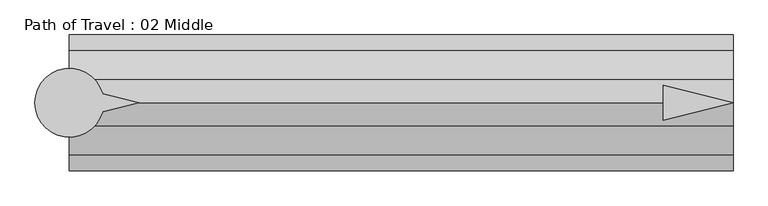
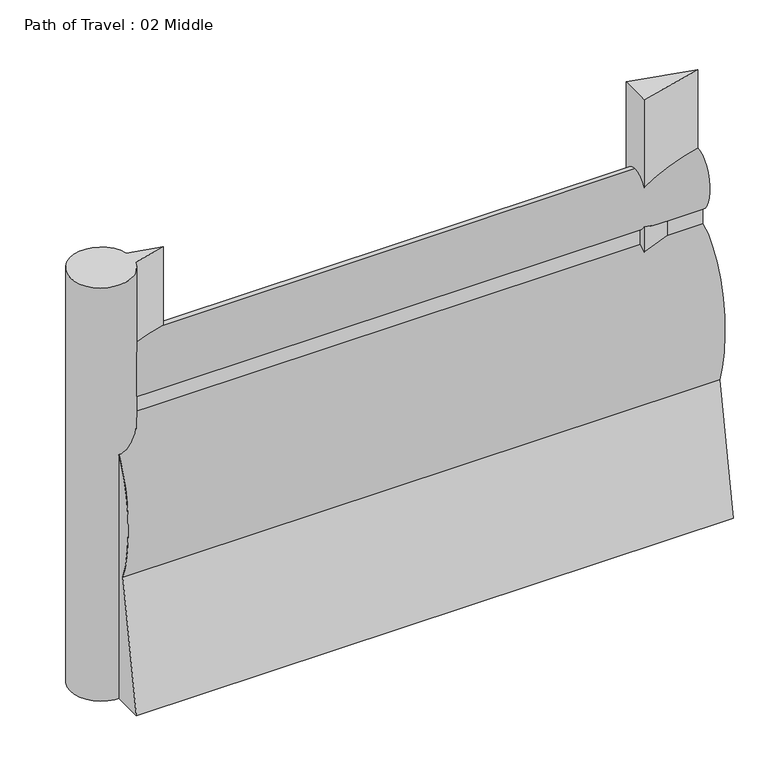
"""IFC4 building model written with IfcOpenShell, lengths in millimetres: proxy geometry, Path of Travel : 02 Middle."""

from ifc_helpers import new_model, si_unit, point, frame, frame_2d, origin, origin_with_axes, place, context, project, spatial, polyline, circle_curve, ellipse_curve, trimmed, segment, composite_curve, outline, extrude, source, transform, mapped, element, save
from ifc_brep_helpers import plane_surface, extruded_surface, advanced_brep


def path_of_travel_02_middle_ce9169e8(model_context):
    return source(origin(), model_context, "Body", "SolidModel", [
        advanced_brep(
        [(227.5554837, 0.0, 1727.2), (227.5554837, 42.9018657, 1436.6534209), (227.5554837, 42.9018657, 1363.4763406), (227.5554837, 184.1186263, 643.4144547), (227.5554837, 297.5699544, 0.0), (227.5554837, 145.6574193, 0.0), (227.5554837, 0.0, 584.2), (227.5554837, -145.6574193, 0.0), (227.5554837, -297.5699544, 0.0), (227.5554837, -184.1186263, 643.4144547), (227.5554837, -42.9018657, 1363.4763406), (227.5554837, -42.9018657, 1436.6534209), (3136.9986776, 0.0, 1727.2), (3136.9986776, -42.9018657, 1436.6534209), (3136.9986776, -42.9018657, 1363.4763406), (3136.9986776, -184.1186263, 643.4144547), (3136.9986776, -297.5699544, 0.0), (3136.9986776, -145.6574193, 0.0), (3136.9986776, 0.0, 584.2), (3136.9986776, 145.6574193, 0.0), (3136.9986776, 297.5699544, 0.0), (3136.9986776, 184.1186263, 643.4144547), (3136.9986776, 42.9018657, 1363.4763406), (3136.9986776, 42.9018657, 1436.6534209)],
        [
            (0, 1, ellipse_curve(frame((227.5554837, 0.0, 1574.8), z_axis=(-1.0, 0.0, 0.0), x_axis=(0.0, 0.0, 1.0)), 152.4, 101.6)),
            (1, 2),
            (2, 3, ellipse_curve(frame((227.5554837, 0.0, 914.4), z_axis=(-1.0, 0.0, 0.0), x_axis=(0.0, 0.0, -1.0)), 457.2, 228.6)),
            (3, 4),
            (4, 5),
            (5, 6),
            (6, 7),
            (7, 8),
            (8, 9),
            (9, 10, ellipse_curve(frame((227.5554837, 0.0, 914.4), z_axis=(-1.0, 0.0, 0.0), x_axis=(0.0, 0.0, -1.0)), 457.2, 228.6)),
            (10, 11),
            (11, 0, ellipse_curve(frame((227.5554837, 0.0, 1574.8), z_axis=(-1.0, 0.0, 0.0), x_axis=(0.0, 0.0, 1.0)), 152.4, 101.6)),
            (12, 13, ellipse_curve(frame((3136.9986776, 0.0, 1574.8), z_axis=(1.0, 0.0, 0.0), x_axis=(0.0, 0.0, 1.0)), 152.4, 101.6)),
            (13, 14),
            (14, 15, ellipse_curve(frame((3136.9986776, 0.0, 914.4), z_axis=(1.0, 0.0, 0.0), x_axis=(0.0, 0.0, -1.0)), 457.2, 228.6)),
            (15, 16),
            (16, 17),
            (17, 18),
            (18, 19),
            (19, 20),
            (20, 21),
            (21, 22, ellipse_curve(frame((3136.9986776, 0.0, 914.4), z_axis=(1.0, 0.0, 0.0), x_axis=(0.0, 0.0, -1.0)), 457.2, 228.6)),
            (22, 23),
            (23, 12, ellipse_curve(frame((3136.9986776, 0.0, 1574.8), z_axis=(1.0, 0.0, 0.0), x_axis=(0.0, 0.0, 1.0)), 152.4, 101.6)),
            (0, 12),
            (23, 1),
            (22, 2),
            (21, 3),
            (20, 4),
            (19, 5),
            (18, 6),
            (17, 7),
            (16, 8),
            (15, 9),
            (14, 10),
            (13, 11),
        ],
        [
            plane_surface(frame((227.5554837, 0.0, 0.0), z_axis=(-1.0, 0.0, 0.0), x_axis=(0.0, 0.0, 1.0))),
            plane_surface(frame((3136.9986776, 0.0, 0.0), z_axis=(1.0, 0.0, 0.0), x_axis=(0.0, 0.0, 1.0))),
            extruded_surface(trimmed(ellipse_curve(frame((3136.9986776, 0.0, 1574.8), z_axis=(-1.0, 0.0, 0.0), x_axis=(0.0, 0.0, 1.0)), 152.4, 101.6), [point((3136.9986776, 0.0, 1727.2))], [point((3136.9986776, 42.9018657, 1436.6534209))], True, "CARTESIAN"), (-2909.4431939, 0.0, 0.0), 2909.4431939),
            plane_surface(frame((227.5554837, 42.9018657, 1436.6534209), z_axis=(0.0, 1.0, 0.0), x_axis=(1.0, 0.0, 0.0))),
            extruded_surface(trimmed(ellipse_curve(frame((3136.9986776, 0.0, 914.4), z_axis=(-1.0, 0.0, 0.0), x_axis=(0.0, 0.0, -1.0)), 457.2, 228.6), [point((3136.9986776, 42.9018657, 1363.4763406))], [point((3136.9986776, 184.1186263, 643.4144547))], True, "CARTESIAN"), (-2909.4431939, 0.0, 0.0), 2909.4431939),
            plane_surface(frame((227.5554837, 184.1186263, 643.4144547), z_axis=(0.0, 0.9848077530122078, 0.1736481776669322), x_axis=(1.0, 0.0, 0.0))),
            plane_surface(frame((227.5554837, 297.5699544, 0.0), z_axis=(0.0, 0.0, -1.0), x_axis=(1.0, 0.0, 0.0))),
            plane_surface(frame((227.5554837, 145.6574193, 0.0), z_axis=(0.0, -0.9702957262760199, -0.2419218955995739), x_axis=(1.0, 0.0, 0.0))),
            plane_surface(frame((227.5554837, 0.0, 584.2), z_axis=(0.0, 0.9702957262759961, -0.24192189559966923), x_axis=(1.0, 0.0, 0.0))),
            plane_surface(frame((227.5554837, -145.6574193, 0.0), z_axis=(0.0, 0.0, -1.0), x_axis=(1.0, 0.0, 0.0))),
            plane_surface(frame((227.5554837, -297.5699544, 0.0), z_axis=(0.0, -0.984807753012208, 0.17364817766693066), x_axis=(1.0, 0.0, 0.0))),
            extruded_surface(trimmed(ellipse_curve(frame((3136.9986776, 0.0, 914.4), z_axis=(-1.0, 0.0, 0.0), x_axis=(0.0, 0.0, -1.0)), 457.2, 228.6), [point((3136.9986776, -184.1186263, 643.4144547))], [point((3136.9986776, -42.9018657, 1363.4763406))], True, "CARTESIAN"), (-2909.4431939, 0.0, 0.0), 2909.4431939),
            plane_surface(frame((227.5554837, -42.9018657, 1363.4763406), z_axis=(0.0, -1.0, 0.0), x_axis=(1.0, 0.0, 0.0))),
            extruded_surface(trimmed(ellipse_curve(frame((3136.9986776, 0.0, 1574.8), z_axis=(-1.0, 0.0, 0.0), x_axis=(0.0, 0.0, 1.0)), 152.4, 101.6), [point((3136.9986776, -42.9018657, 1436.6534209))], [point((3136.9986776, 0.0, 1727.2))], True, "CARTESIAN"), (-2909.4431939, 0.0, 0.0), 2909.4431939),
        ],
        [
            (0, [[1, 2, 3, 4, 5, 6, 7, 8, 9, 10, 11, 12]]),
            (1, [[13, 14, 15, 16, 17, 18, 19, 20, 21, 22, 23, 24]]),
            (2, [[-1, 25, -24, 26]]),
            (3, [[-2, -26, -23, 27]]),
            (4, [[-3, -27, -22, 28]]),
            (5, [[-4, -28, -21, 29]]),
            (6, [[-5, -29, -20, 30]]),
            (7, [[-6, -30, -19, 31]]),
            (8, [[-7, -31, -18, 32]]),
            (9, [[-8, -32, -17, 33]]),
            (10, [[-9, -33, -16, 34]]),
            (11, [[-10, -34, -15, 35]]),
            (12, [[-11, -35, -14, 36]]),
            (13, [[-12, -36, -13, -25]]),
        ],
    ),
        extrude(outline(polyline([(2830.9935311, 76.2006338), (3136.9986776, 0.0), (2830.9935311, -76.2006338), (2830.9935311, 76.2006338)])), origin_with_axes(), (0.0, 0.0, 1.0), 2129.5973753),
        extrude(outline(composite_curve([segment(polyline([(372.7837828, 39.4440225), (531.182385, 0.0), (372.7837828, -39.4440225)]), True, "CONTINUOUS"), segment(trimmed(circle_curve(frame_2d((227.2200886, 0.0)), 150.8131956), [point((372.7837828, -39.4440225))], [point((372.7837828, 39.4440225))], False, "CARTESIAN"), True, "CONTINUOUS")], self_intersect=False)), origin_with_axes(), (0.0, 0.0, 1.0), 2129.5973753),
    ])


if __name__ == "__main__":
    model = new_model("IFC4")
    model_context = context("Model", 3, world=origin())
    ifc_project = project(units=[si_unit("LENGTHUNIT", "METRE", prefix="MILLI")], contexts=[model_context])
    site = spatial("IfcSite", under=ifc_project)
    building = spatial("IfcBuilding", under=site)
    placement = place(None, origin())
    path_of_travel_02_middle_shape = path_of_travel_02_middle_ce9169e8(model_context)
    element("IfcBuildingElementProxy", 1, Name="Path of Travel : 02 Middle", ObjectType="Path of Travel : 02 Middle", at=placement, inside=building, context=model_context, shape_type="MappedRepresentation", body=[
        mapped(path_of_travel_02_middle_shape, transform((0.0, 0.0, 0.0), x_axis=(1.0, 0.0, 0.0), y_axis=(0.0, 1.0, 0.0), z_axis=(0.0, 0.0, 1.0))),
    ])
    save(model, "model.ifc")

# Revit data of these elements
# Type "Path of Travel : 02 Middle"
#   Path of Egress [instance default] = 4' - 0"
#   built-in parameter 1001306 [instance default] = 4 (stored number, unit not read)
#   Dot at Start = no
#   Arrow in Middle = yes
#   Arrow at End = no
#   Egress Path = none
# Element 1 (IfcBuildingElementProxy, "Path of Travel : 02 Middle")
#   Path of Egress = 9' - 6.54501"
#   built-in parameter 1001306 = 9.54542 (stored number, unit not read)
